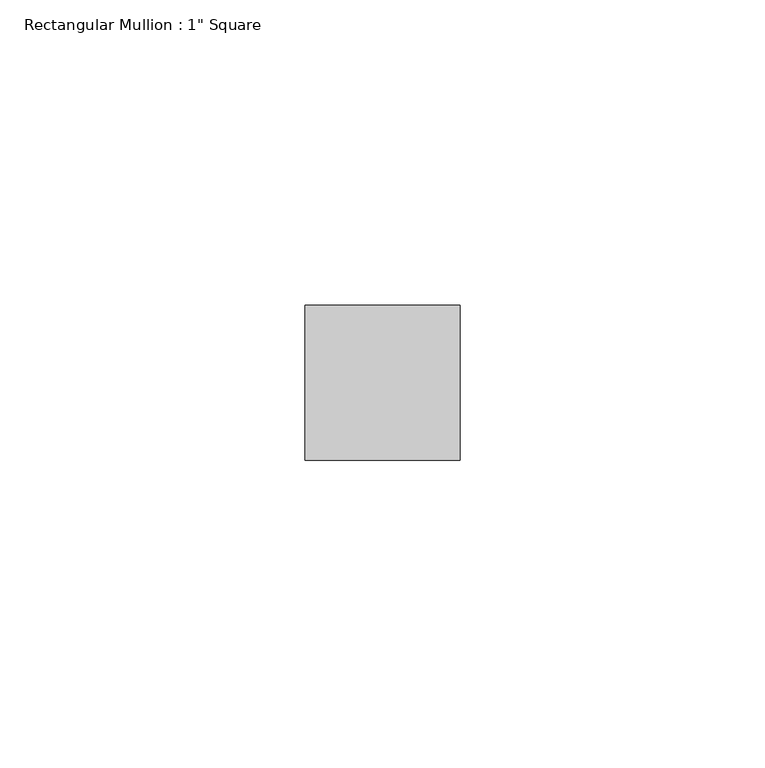
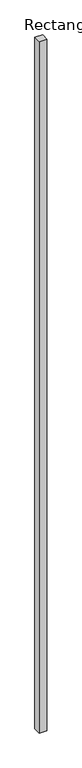
"""IFC4 building model written with IfcOpenShell, lengths in millimetres: member geometry."""

import ifcopenshell
import ifcopenshell.guid

model = None  # the IFC model being written
_history = None  # IfcOwnerHistory: only IFC2X3 demands one
_inside = {}  # id of a spatial element -> (the spatial element, [elements in it])
_under = {}  # id of a project, library or spatial element -> (it, [spatial elements below it])
_declared = {}  # id of a project -> (the project, [libraries it declares])
_typed = {}  # id of a type object -> (the type object, [elements of that type])
_made_of = {}  # id of a material, layer set ... -> (it, [elements and type objects made of it])


def new_model(schema):
    """Start an empty IFC model of exactly this schema.

    Asked for "IFC4X3", IfcOpenShell would pick the latest addendum, in which some entities
    have other attributes; the version numbers below select the first issue.
    IFC2X3 requires an IfcOwnerHistory on every rooted entity: one is made here for all.
    """
    global model, _history
    if schema == "IFC4X3":
        model = ifcopenshell.file(schema_version=(4, 3, 0, 0))
    else:
        model = ifcopenshell.file(schema=schema)
    _inside.clear()
    _under.clear()
    _declared.clear()
    _typed.clear()
    _made_of.clear()
    _history = None
    if model.schema == "IFC2X3":
        org = make("IfcOrganization", Name="unknown")
        user = make(
            "IfcPersonAndOrganization",
            ThePerson=make("IfcPerson", FamilyName="unknown"),
            TheOrganization=org,
        )
        app = make(
            "IfcApplication",
            ApplicationDeveloper=org,
            Version="unknown",
            ApplicationFullName="unknown",
            ApplicationIdentifier="unknown",
        )
        _history = make(
            "IfcOwnerHistory",
            OwningUser=user,
            OwningApplication=app,
            ChangeAction="ADDED",
            CreationDate=0,
        )
    return model


def make(cls, **values):
    """One entity of the class cls with the attributes given. An attribute that is None is left unset."""
    return model.create_entity(
        cls, **{name: value for name, value in values.items() if value is not None}
    )


def rooted(cls, **values):
    """An entity with a GlobalId (a new one), such as an element, a storey or a relation."""
    return make(cls, GlobalId=ifcopenshell.guid.new(), OwnerHistory=_history, **values)


def si_unit(unit_type, name, prefix=None):
    """IfcSIUnit, for example si_unit("LENGTHUNIT", "METRE", prefix="MILLI")."""
    return make("IfcSIUnit", UnitType=unit_type, Prefix=prefix, Name=name)


def assignment(units):
    """IfcUnitAssignment: the units of a project."""
    return None if units is None else make("IfcUnitAssignment", Units=units)


def point(xyz):
    """IfcCartesianPoint."""
    return None if xyz is None else make("IfcCartesianPoint", Coordinates=xyz)


def direction(xyz):
    """IfcDirection."""
    return None if xyz is None else make("IfcDirection", DirectionRatios=xyz)


def frame(location, z_axis=None, x_axis=None):
    """IfcAxis2Placement3D, a coordinate frame: its origin and axes. An axis left out is left unset."""
    return make(
        "IfcAxis2Placement3D",
        Location=point(location),
        Axis=direction(z_axis),
        RefDirection=direction(x_axis),
    )


def origin():
    """The frame at (0, 0, 0) with its axes left unset."""
    return frame((0.0, 0.0, 0.0))


def place(relative_to, where):
    """IfcLocalPlacement: puts the frame where relative to a parent placement (None: the world)."""
    return make(
        "IfcLocalPlacement", PlacementRelTo=relative_to, RelativePlacement=where
    )


def context(
    kind, dimensions, precision=None, world=None, true_north=None, identifier=None
):
    """IfcGeometricRepresentationContext, for example the 3D "Model" context."""
    return make(
        "IfcGeometricRepresentationContext",
        ContextIdentifier=identifier,
        ContextType=kind,
        CoordinateSpaceDimension=dimensions,
        Precision=precision,
        WorldCoordinateSystem=world,
        TrueNorth=true_north,
    )


def project(units=None, contexts=None):
    """IfcProject with its units and contexts."""
    return rooted(
        "IfcProject",
        Name="project",
        RepresentationContexts=contexts,
        UnitsInContext=assignment(units),
    )


def spatial(cls, under=None, at=None, **own):
    """A site, building, storey or space (cls), placed at a placement, below another one or the project."""
    s = rooted(cls, ObjectPlacement=at, **own)
    if under is not None:
        _under.setdefault(under.id(), (under, []))[1].append(s)
    return s


def polyline(points):
    """IfcPolyline through the points."""
    return make("IfcPolyline", Points=[point(p) for p in points])


def outline(outer, holes=None, kind="AREA"):
    """IfcArbitraryClosedProfileDef: a profile drawn as a closed curve; with holes, ...WithVoids."""
    if holes is None:
        return make("IfcArbitraryClosedProfileDef", ProfileType=kind, OuterCurve=outer)
    return make(
        "IfcArbitraryProfileDefWithVoids",
        ProfileType=kind,
        OuterCurve=outer,
        InnerCurves=holes,
    )


def extrude(swept, where, along, depth):
    """IfcExtrudedAreaSolid: the profile swept, set in the frame where, extruded along a direction by depth."""
    return make(
        "IfcExtrudedAreaSolid",
        SweptArea=swept,
        Position=where,
        ExtrudedDirection=direction(along),
        Depth=depth,
    )


def shape(context_of_items, identifier, shape_type, items):
    """IfcShapeRepresentation: the items that make up one representation, for example the "Body"."""
    return make(
        "IfcShapeRepresentation",
        ContextOfItems=context_of_items,
        RepresentationIdentifier=identifier,
        RepresentationType=shape_type,
        Items=items,
    )


def source(mapping_origin, context_of_items, identifier, shape_type, items):
    """IfcRepresentationMap: a shape defined once, which mapped items show again and again."""
    return make(
        "IfcRepresentationMap",
        MappingOrigin=mapping_origin,
        MappedRepresentation=shape(context_of_items, identifier, shape_type, items),
    )


def transform(
    local_origin,
    x_axis=None,
    y_axis=None,
    z_axis=None,
    scale=None,
    scale2=None,
    scale3=None,
    uniform=True,
):
    """IfcCartesianTransformationOperator3D, or its non-uniform kind. x_axis, y_axis, z_axis: its Axis1, 2, 3."""
    if uniform:
        return make(
            "IfcCartesianTransformationOperator3D",
            Axis1=direction(x_axis),
            Axis2=direction(y_axis),
            LocalOrigin=point(local_origin),
            Scale=scale,
            Axis3=direction(z_axis),
        )
    return make(
        "IfcCartesianTransformationOperator3DnonUniform",
        Axis1=direction(x_axis),
        Axis2=direction(y_axis),
        LocalOrigin=point(local_origin),
        Scale=scale,
        Axis3=direction(z_axis),
        Scale2=scale2,
        Scale3=scale3,
    )


def mapped(mapping_source, mapping_target):
    """IfcMappedItem: shows the shape of a source again, moved by a transform."""
    return make(
        "IfcMappedItem", MappingSource=mapping_source, MappingTarget=mapping_target
    )


def made_of(thing, what):
    """Note that an element or type object is made of a material, layer set ...; save() writes the relation."""
    if what is not None:
        _made_of.setdefault(what.id(), (what, []))[1].append(thing)
    return thing


def element(
    cls,
    number,
    at=None,
    inside=None,
    cuts=None,
    type_object=None,
    material=None,
    context=None,
    identifier="Body",
    shape_type=None,
    held_by="IfcProductDefinitionShape",
    body=None,
    shapes=None,
    **own,
):
    """One element of the class cls, such as IfcWall. Its Tag is "e" and its number.

    at: its placement. inside: the storey or other place that contains it. cuts: it is an
    opening in that element (IfcRelVoidsElement). A single representation is given by context,
    identifier, shape_type and body (its items); several are given by shapes. held_by: the class
    of the entity that holds the representations. save() writes the other relations.
    """
    e = rooted(cls, Tag="e%d" % number, ObjectPlacement=at, **own)
    if body is not None:
        shapes = [shape(context, identifier, shape_type, body)]
    if shapes is not None:
        e.Representation = make(held_by, Representations=shapes)
    if inside is not None:
        _inside.setdefault(inside.id(), (inside, []))[1].append(e)
    if cuts is not None:
        rooted(
            "IfcRelVoidsElement", RelatingBuildingElement=cuts, RelatedOpeningElement=e
        )
    if type_object is not None:
        _typed.setdefault(type_object.id(), (type_object, []))[1].append(e)
    return made_of(e, material)


def aggregate(whole, parts):
    """IfcRelAggregates: a whole, such as a stair, and the parts it consists of."""
    return rooted("IfcRelAggregates", RelatingObject=whole, RelatedObjects=parts)


def save(model, path):
    """Write the relations noted so far, then the file.

    IfcRelAggregates (storeys below a building ...), IfcRelContainedInSpatialStructure (elements
    in a storey), IfcRelDefinesByType, IfcRelAssociatesMaterial and IfcRelDeclares: one each for
    every whole, place, type object, material and project.
    """
    for whole, parts in _under.values():
        aggregate(whole, parts)
    for where, things in _inside.values():
        rooted(
            "IfcRelContainedInSpatialStructure",
            RelatedElements=things,
            RelatingStructure=where,
        )
    for kind, things in _typed.values():
        rooted("IfcRelDefinesByType", RelatedObjects=things, RelatingType=kind)
    for what, things in _made_of.values():
        rooted("IfcRelAssociatesMaterial", RelatedObjects=things, RelatingMaterial=what)
    for by, libraries in _declared.values():
        rooted("IfcRelDeclares", RelatingContext=by, RelatedDefinitions=libraries)
    model.write(path)


def member_f92d9b35(model_context):
    return source(origin(), model_context, "Body", "SweptSolid", [
        extrude(outline(polyline([(0.0, 12.7), (0.0, -12.7), (-25.4, -12.7), (-25.4, 12.7), (0.0, 12.7)])), frame((0.0, 0.0, -2438.4), z_axis=(0.0, 0.0, 1.0), x_axis=(1.0, 0.0, 0.0)), (0.0, 0.0, 1.0), 2438.4),
    ])


if __name__ == "__main__":
    model = new_model("IFC4")
    model_context = context("Model", 3, world=origin())
    ifc_project = project(units=[si_unit("LENGTHUNIT", "METRE", prefix="MILLI")], contexts=[model_context])
    site = spatial("IfcSite", under=ifc_project)
    building = spatial("IfcBuilding", under=site)
    placement = place(None, origin())
    member_shape = member_f92d9b35(model_context)
    element("IfcMember", 1, ObjectType="Rectangular Mullion : 1\" Square", at=placement, inside=building, context=model_context, shape_type="MappedRepresentation", body=[
        mapped(member_shape, transform((0.0, 0.0, 0.0), x_axis=(1.0, 0.0, 0.0), y_axis=(0.0, 1.0, 0.0), z_axis=(0.0, 0.0, 1.0))),
    ])
    save(model, "model.ifc")

# Revit data of these elements
# Type "Rectangular Mullion : 1\" Square"
#   built-in parameter 1007304 = 0.0833333 (stored number, unit not read)
#   built-in parameter 1007301 = 0.0416667 (stored number, unit not read)
#   built-in parameter 1007300 = 0.0416667 (stored number, unit not read)
# Element 1 (IfcMember, "Rectangular Mullion : 1\" Square")
#   Materials on its faces: "Metal - Aluminum"
# Materials
#   "Metal - Aluminum": class "Metal", colour RGB 247 247 247, transparency 0
